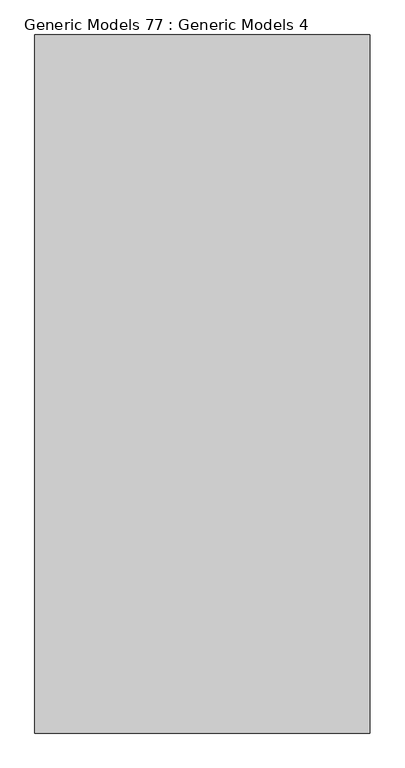
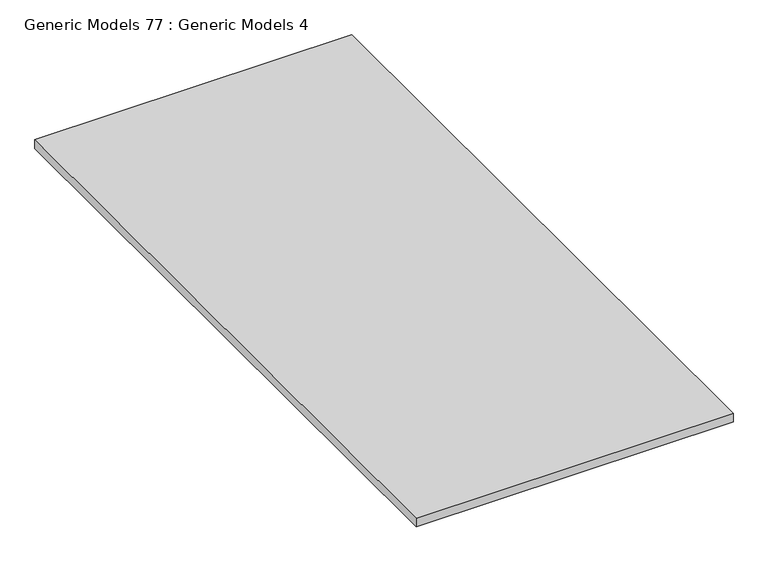
"""IFC4 building model written with IfcOpenShell, lengths in millimetres: proxy geometry, Generic Models 77 : Generic Models 4."""

from ifc_helpers import new_model, si_unit, frame, origin, place, context, project, spatial, polyline, outline, extrude, source, transform, mapped, element, save


def generic_models_77_generic_models_4_d9d10128(model_context):
    return source(origin(), model_context, "Body", "SweptSolid", [
        extrude(outline(polyline([(24896.3074258, -7845.1058743), (24896.3074258, -11442.9554199), (23168.0573109, -11442.9554199), (23168.0573109, -7845.1058743), (24896.3074258, -7845.1058743)])), frame((0.0, 0.0, 123057.2484874), z_axis=(0.0, 0.0, 1.0), x_axis=(1.0, 0.0, 0.0)), (0.0, 0.0, 1.0), 50.8),
    ])


if __name__ == "__main__":
    model = new_model("IFC4")
    model_context = context("Model", 3, world=origin())
    ifc_project = project(units=[si_unit("LENGTHUNIT", "METRE", prefix="MILLI")], contexts=[model_context])
    site = spatial("IfcSite", under=ifc_project)
    building = spatial("IfcBuilding", under=site)
    placement = place(None, origin())
    generic_models_77_generic_models_4_shape = generic_models_77_generic_models_4_d9d10128(model_context)
    element("IfcBuildingElementProxy", 1, Name="Generic Models 77 : Generic Models 4", ObjectType="Generic Models 77 : Generic Models 4", at=placement, inside=building, context=model_context, shape_type="MappedRepresentation", body=[
        mapped(generic_models_77_generic_models_4_shape, transform((0.0, 0.0, 0.0), x_axis=(1.0, 0.0, 0.0), y_axis=(0.0, 1.0, 0.0), z_axis=(0.0, 0.0, 1.0))),
    ])
    save(model, "model.ifc")

# Revit data of these elements
# Element 1 (IfcBuildingElementProxy, "Generic Models 77 : Generic Models 4")
#   Materials on its faces: "_2\" SAND"
# Materials
#   "_2\" SAND": class "Generic", colour RGB 245 226 173, transparency 0, Cost = 0
